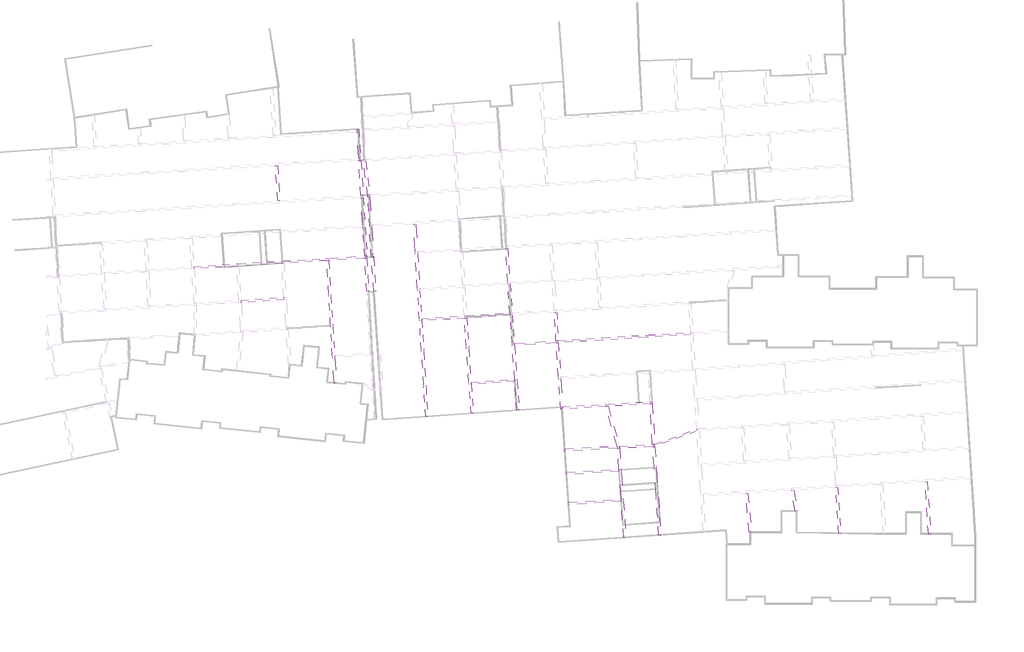
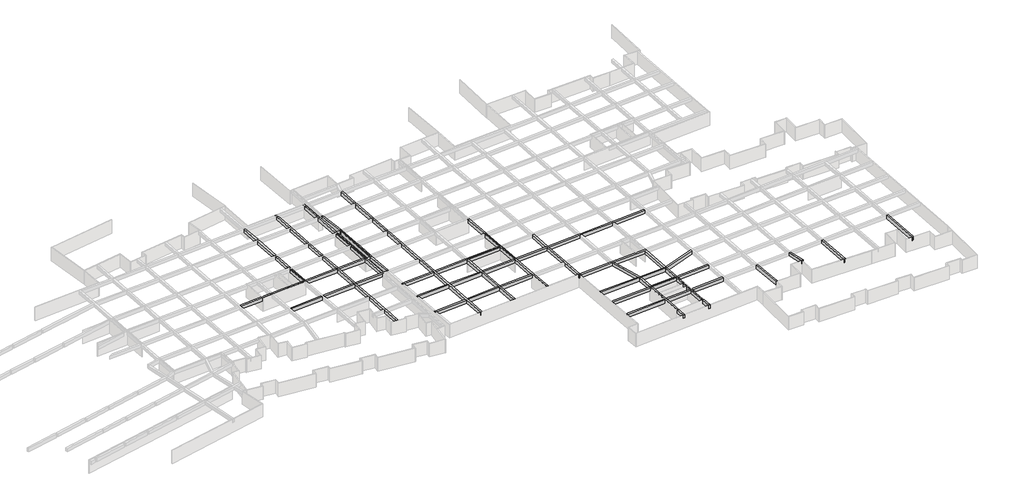
# One storey, part 12 of 14: 33 beams.
"""IFC4 building model written with IfcOpenShell, lengths in millimetres."""

from ifc_helpers import new_model, si_unit, frame, origin, place, context, project, spatial, polyline, outline, extrude, faceted_brep, element, save

model = new_model("IFC4")

# Units and contexts
model_context = context("Model", 3, world=origin())
ifc_project = project(units=[si_unit("LENGTHUNIT", "METRE", prefix="MILLI")], contexts=[model_context])

# Site, building, storey
site = spatial("IfcSite", under=ifc_project)
building = spatial("IfcBuilding", under=site)
storey = spatial("IfcBuildingStorey", under=building, Name="户型图", Elevation=0.0)

# Beams
placement = place(None, origin())
element("IfcBeam", 1, ObjectType="混凝土 - 矩形梁 : KL_beam", at=placement, inside=storey, context=model_context, shape_type="Brep", body=[
    faceted_brep([(-168844.3273357, -151421.9591856, 3300.0), (-168818.123542, -151821.1019553, 3300.0), (-161243.2908554, -151347.7846852, 3300.0), (-160844.0689153, -151322.8390994, 3300.0), (-153230.0656261, -150847.0742344, 3300.0), (-152830.8332777, -150822.1279982, 3300.0), (-145215.8086802, -150346.2993162, 3300.0), (-144816.5872887, -150321.3537646, 3300.0), (-138446.7291671, -149923.3299427, 3300.0), (-138047.4968186, -149898.3837065, 3300.0), (-138061.4513517, -149698.8245855, 3300.0), (-138075.4001739, -149499.3471348, 3300.0), (-138410.3239769, -149520.2750189, 3300.0), (-144841.5328402, -149922.1323731, 3300.0), (-145240.7542318, -149947.0779246, 3300.0), (-152857.2632096, -150422.9993589, 3300.0), (-153256.4846011, -150447.9449104, 3300.0), (-160869.6763174, -150923.659064, 3300.0), (-161268.8982576, -150948.6046498, 3300.0), (-138047.4968186, -149898.3837065, 2500.0), (-168818.123542, -151821.1019553, 2500.0), (-161243.2908554, -151347.7846852, 2500.0), (-160844.0689153, -151322.8390994, 2500.0), (-153230.0656261, -150847.0742344, 2500.0), (-152830.8332777, -150822.1279982, 2500.0), (-145215.8086802, -150346.2993162, 2500.0), (-144816.5872887, -150321.3537646, 2500.0), (-138446.7291671, -149923.3299427, 2500.0), (-168844.3273357, -151421.9591856, 2500.0), (-161268.8982576, -150948.6046498, 2500.0), (-160869.6763174, -150923.659064, 2500.0), (-153256.4846011, -150447.9449104, 2500.0), (-152857.2632096, -150422.9993589, 2500.0), (-145240.7542318, -149947.0779246, 2500.0), (-144841.5328402, -149922.1323731, 2500.0), (-138410.3239769, -149520.2750189, 2500.0), (-138075.4001739, -149499.3471348, 2500.0), (-138061.4513517, -149698.8245855, 2500.0)], [[[0, 1, 2, 3, 4, 5, 6, 7, 8, 9, 10, 11, 12, 13, 14, 15, 16, 17, 18]], [[19, 9, 8, 7, 6, 5, 4, 3, 2, 1, 20, 21, 22, 23, 24, 25, 26, 27]], [[20, 28, 29, 30, 31, 32, 33, 34, 35, 36, 37, 19, 27, 26, 25, 24, 23, 22, 21]], [[28, 0, 18, 17, 16, 15, 14, 13, 12, 11, 36, 35, 34, 33, 32, 31, 30, 29]], [[0, 28, 20, 1]], [[11, 10, 9, 19, 37, 36]]]),
])
element("IfcBeam", 2, ObjectType="混凝土 - 矩形梁 : KL_beam", at=placement, inside=storey, context=model_context, shape_type="SweptSolid", body=[
    extrude(outline(polyline([(-152857.2632096, -150422.9993589), (-153256.4846011, -150447.9449104), (-153570.081579, -145429.2295811), (-153170.8601875, -145404.2840296), (-152857.2632096, -150422.9993589)])), frame((0.0, 0.0, 2500.0), z_axis=(0.0, 0.0, 1.0), x_axis=(1.0, 0.0, 0.0)), (0.0, 0.0, 1.0), 800.0),
    extrude(outline(polyline([(-154632.6280549, -128424.5431139), (-154233.4066634, -128399.5975624), (-153944.0174942, -133030.8981222), (-154343.2012363, -133056.4462052), (-154632.6280549, -128424.5431139)])), frame((0.0, 0.0, 2500.0), z_axis=(0.0, 0.0, 1.0), x_axis=(1.0, 0.0, 0.0)), (0.0, 0.0, 1.0), 800.0),
    extrude(outline(polyline([(-153902.4547638, -140110.0252686), (-153503.2333722, -140085.079717), (-153195.805739, -145005.062638), (-153595.0271306, -145030.0081896), (-153902.4547638, -140110.0252686)])), frame((0.0, 0.0, 2500.0), z_axis=(0.0, 0.0, 1.0), x_axis=(1.0, 0.0, 0.0)), (0.0, 0.0, 1.0), 800.0),
    extrude(outline(polyline([(-153528.1789238, -139685.8583255), (-153927.4003153, -139710.803877), (-154318.2556563, -133455.6680514), (-153919.0719143, -133430.1199684), (-153528.1789238, -139685.8583255)])), frame((0.0, 0.0, 2500.0), z_axis=(0.0, 0.0, 1.0), x_axis=(1.0, 0.0, 0.0)), (0.0, 0.0, 1.0), 800.0),
])
element("IfcBeam", 3, ObjectType="混凝土 - 矩形梁 : KL_beam", at=placement, inside=storey, context=model_context, shape_type="Brep", body=[
    faceted_brep([(-143451.1806272, -172172.9270426, 3300.0), (-143850.4020187, -172197.8725942, 3300.0), (-143850.4020187, -172197.8725942, 2500.0), (-143451.1806272, -172172.9270426, 2500.0), (-143732.1819625, -167675.8629499, 3300.0), (-143757.1298345, -167276.6044225, 3300.0), (-144078.3820209, -162135.3773504, 3300.0), (-144103.3276067, -161736.1554102, 3300.0), (-144417.0732982, -156715.0601116, 3300.0), (-144442.0195344, -156315.8277631, 3300.0), (-144816.5872887, -150321.3537646, 3300.0), (-145215.8086802, -150346.2993162, 3300.0), (-144841.0561061, -156343.7311184, 3300.0), (-144816.1098699, -156742.9634669, 3300.0), (-144502.5076422, -161761.7628124, 3300.0), (-144477.5620564, -162160.9847526, 3300.0), (-144156.0109682, -167306.995361, 3300.0), (-144131.0630962, -167706.2538884, 3300.0), (-145215.8086802, -150346.2993162, 2500.0), (-144841.0561061, -156343.7311184, 2500.0), (-144816.1098699, -156742.9634669, 2500.0), (-144502.5076422, -161761.7628124, 2500.0), (-144477.5620564, -162160.9847526, 2500.0), (-144156.0109682, -167306.995361, 2500.0), (-144131.0630962, -167706.2538884, 2500.0), (-144816.5872887, -150321.3537646, 2500.0), (-144442.0195344, -156315.8277631, 2500.0), (-144417.0732982, -156715.0601116, 2500.0), (-144103.3276067, -161736.1554102, 2500.0), (-144078.3820209, -162135.3773504, 2500.0), (-143757.1298345, -167276.6044225, 2500.0), (-143732.1819625, -167675.8629499, 2500.0)], [[[0, 1, 2, 3]], [[1, 0, 4, 5, 6, 7, 8, 9, 10, 11, 12, 13, 14, 15, 16, 17]], [[2, 1, 17, 16, 15, 14, 13, 12, 11, 18, 19, 20, 21, 22, 23, 24]], [[3, 2, 24, 23, 22, 21, 20, 19, 18, 25, 26, 27, 28, 29, 30, 31]], [[0, 3, 31, 30, 29, 28, 27, 26, 25, 10, 9, 8, 7, 6, 5, 4]], [[11, 10, 25, 18]]]),
    faceted_brep([(-146252.6907928, -127338.3686664, 3300.0), (-146252.6907928, -127338.3686664, 2500.0), (-146651.9121843, -127363.3142179, 2500.0), (-146651.9121843, -127363.3142179, 3300.0), (-146242.6218456, -127499.509185, 3300.0), (-146641.8432371, -127524.4547366, 3300.0), (-146641.8432371, -127524.4547366, 2500.0), (-146242.6218456, -127499.509185, 2500.0)], [[[0, 1, 2, 3]], [[4, 5, 6, 7]], [[0, 3, 5, 4]], [[3, 2, 6, 5]], [[2, 1, 7, 6]], [[1, 0, 4, 7]]]),
    faceted_brep([(-144841.5328402, -149922.1323731, 3300.0), (-145240.7542318, -149947.0779246, 3300.0), (-145240.7542318, -149947.0779246, 2500.0), (-144841.5328402, -149922.1323731, 2500.0), (-145155.1298182, -144903.4170437, 3300.0), (-145554.3512097, -144928.3625953, 3300.0), (-145554.3512097, -144928.3625953, 2500.0), (-145155.1298182, -144903.4170437, 2500.0)], [[[0, 1, 2, 3]], [[1, 0, 4, 5]], [[2, 1, 5, 6]], [[3, 2, 6, 7]], [[0, 3, 7, 4]], [[5, 4, 7, 6]]]),
    faceted_brep([(-145886.7243944, -139609.1582827, 3300.0), (-145487.5030029, -139584.2127312, 3300.0), (-145487.5030029, -139584.2127312, 2500.0), (-145886.7243944, -139609.1582827, 2500.0), (-145180.0753697, -144504.1956522, 3300.0), (-145579.2967612, -144529.1412037, 3300.0), (-145579.2967612, -144529.1412037, 2500.0), (-145180.0753697, -144504.1956522, 2500.0)], [[[0, 1, 2, 3]], [[4, 5, 6, 7]], [[1, 0, 5, 4]], [[0, 3, 6, 5]], [[3, 2, 7, 6]], [[2, 1, 4, 7]]]),
    faceted_brep([(-145512.4485544, -139184.9913397, 3300.0), (-145911.669946, -139209.9368912, 3300.0), (-145911.669946, -139209.9368912, 2500.0), (-145512.4485544, -139184.9913397, 2500.0), (-145904.0974866, -132917.15511, 3300.0), (-146303.2812287, -132942.703193, 3300.0), (-146303.2812287, -132942.703193, 2500.0), (-145904.0974866, -132917.15511, 2500.0)], [[[0, 1, 2, 3]], [[1, 0, 4, 5]], [[2, 1, 5, 6]], [[3, 2, 6, 7]], [[0, 3, 7, 4]], [[5, 4, 7, 6]]]),
    faceted_brep([(-145929.0430666, -132517.9332638, 3300.0), (-146328.2268086, -132543.4813468, 3300.0), (-146328.2268086, -132543.4813468, 2500.0), (-145929.0430666, -132517.9332638, 2500.0), (-146217.676294, -127898.7305766, 3300.0), (-146616.8976856, -127923.6761281, 3300.0), (-146616.8976856, -127923.6761281, 2500.0), (-146217.676294, -127898.7305766, 2500.0)], [[[0, 1, 2, 3]], [[1, 0, 4, 5]], [[2, 1, 5, 6]], [[3, 2, 6, 7]], [[0, 3, 7, 4]], [[5, 4, 7, 6]]]),
])
element("IfcBeam", 4, ObjectType="混凝土 - 矩形梁 : KL_beam", at=placement, inside=storey, context=model_context, shape_type="Brep", body=[
    faceted_brep([(-137604.1419621, -156238.6535432, 3300.0), (-137632.0445516, -155839.6279231, 3300.0), (-138031.0701717, -155867.5305126, 3300.0), (-144442.0195344, -156315.8277631, 3300.0), (-144417.0732982, -156715.0601116, 3300.0), (-138005.1737883, -156266.6964203, 3300.0), (-137606.1281956, -156238.7924342, 3300.0), (-137604.1419621, -156238.6535432, 2500.0), (-144417.0732982, -156715.0601116, 2500.0), (-138005.1737883, -156266.6964203, 2500.0), (-137606.1281956, -156238.7924342, 2500.0), (-137632.0445516, -155839.6279231, 2500.0), (-144442.0195344, -156315.8277631, 2500.0), (-138031.0701717, -155867.5305126, 2500.0)], [[[0, 1, 2, 3, 4, 5, 6]], [[7, 0, 6, 5, 4, 8, 9, 10]], [[11, 7, 10, 9, 8, 12, 13]], [[1, 11, 13, 12, 3, 2]], [[4, 3, 12, 8]], [[1, 0, 7, 11]]]),
    faceted_brep([(-160426.3434263, -157834.5373332, 3300.0), (-160451.9512168, -157435.3512451, 3300.0), (-160451.9512168, -157435.3512451, 2500.0), (-160426.3434263, -157834.5373332, 2500.0), (-152806.7516024, -156900.7468094, 3300.0), (-152778.8490129, -157299.7724295, 3300.0), (-152778.8490129, -157299.7724295, 2500.0), (-152806.7516024, -156900.7468094, 2500.0)], [[[0, 1, 2, 3]], [[4, 5, 6, 7]], [[1, 0, 5, 4]], [[0, 3, 6, 5]], [[3, 2, 7, 6]], [[2, 1, 4, 7]]]),
    faceted_brep([(-152379.8233928, -157271.86984, 3300.0), (-152407.7259823, -156872.8442199, 3300.0), (-152407.7259823, -156872.8442199, 2500.0), (-152379.8233928, -157271.86984, 2500.0), (-144841.0561061, -156343.7311184, 3300.0), (-144816.1098699, -156742.9634669, 3300.0), (-144816.1098699, -156742.9634669, 2500.0), (-144841.0561061, -156343.7311184, 2500.0)], [[[0, 1, 2, 3]], [[4, 5, 6, 7]], [[1, 0, 5, 4]], [[0, 3, 6, 5]], [[3, 2, 7, 6]], [[2, 1, 4, 7]]]),
])
element("IfcBeam", 5, ObjectType="混凝土 - 矩形梁 : KL_beam", at=placement, inside=storey, context=model_context, shape_type="SweptSolid", body=[
    extrude(outline(polyline([(-139472.272293, -132525.1613278), (-139073.0509015, -132500.2157763), (-138682.0182996, -138758.1884339), (-139081.2396911, -138783.1339854), (-139472.272293, -132525.1613278)])), frame((0.0, 0.0, 2500.0), z_axis=(0.0, 0.0, 1.0), x_axis=(1.0, 0.0, 0.0)), (0.0, 0.0, 1.0), 800.0),
])
element("IfcBeam", 6, ObjectType="混凝土 - 矩形梁 : KL_beam", at=placement, inside=storey, context=model_context, shape_type="Brep", body=[
    faceted_brep([(-138257.4280169, -132256.5266916, 3300.0), (-138654.6809564, -132303.3252176, 3300.0), (-137889.4671884, -138798.902005, 3300.0), (-137866.6756453, -138992.369798, 3300.0), (-137478.1152384, -138968.0904035, 3300.0), (-137466.852736, -138967.3866603, 3300.0), (-137513.7217746, -138569.535169, 3300.0), (-138210.5692457, -132654.2910271, 3300.0), (-138654.6809564, -132303.3252176, 2500.0), (-137889.4671884, -138798.902005, 2500.0), (-137866.6756453, -138992.369798, 2500.0), (-138257.4280169, -132256.5266916, 2500.0), (-138210.5692457, -132654.2910271, 2500.0), (-137513.7217746, -138569.535169, 2500.0), (-137466.852736, -138967.3866603, 2500.0), (-137478.1152384, -138968.0904035, 2500.0)], [[[0, 1, 2, 3, 4, 5, 6, 7]], [[1, 8, 9, 10, 3, 2]], [[8, 11, 12, 13, 14, 15, 10, 9]], [[11, 0, 7, 6, 5, 14, 13, 12]], [[0, 11, 8, 1]], [[5, 4, 3, 10, 15, 14]]]),
])
element("IfcBeam", 7, ObjectType="混凝土 - 矩形梁 : KL_beam", at=placement, inside=storey, context=model_context, shape_type="SweptSolid", body=[
    extrude(outline(polyline([(-138446.7291671, -149923.3299427), (-138047.4968186, -149898.3837065), (-137632.0445516, -155839.6279231), (-138031.0701717, -155867.5305126), (-138446.7291671, -149923.3299427)])), frame((0.0, 0.0, 2500.0), z_axis=(0.0, 0.0, 1.0), x_axis=(1.0, 0.0, 0.0)), (0.0, 0.0, 1.0), 800.0),
])
element("IfcBeam", 8, ObjectType="混凝土 - 矩形梁 : KL_beam", at=placement, inside=storey, context=model_context, shape_type="Brep", body=[
    faceted_brep([(-136817.1755094, -149686.5252144, 3300.0), (-136817.1755094, -149686.5252144, 2500.0), (-137207.4432782, -149713.8153953, 2500.0), (-137216.2011295, -149714.4278039, 2500.0), (-137216.2011295, -149714.4278039, 3300.0), (-137207.4432782, -149713.8153953, 3300.0), (-136785.0174146, -155880.6422056, 3300.0), (-136385.9917945, -155852.7396161, 3300.0), (-136805.9297538, -149847.3470126, 3300.0), (-136785.0174146, -155880.6422056, 2500.0), (-136805.9297538, -149847.3470126, 2500.0), (-136385.9917945, -155852.7396161, 2500.0)], [[[0, 1, 2, 3, 4, 5]], [[0, 5, 4, 6, 7, 8]], [[4, 3, 9, 6]], [[3, 2, 1, 10, 11, 9]], [[1, 0, 8, 7, 11, 10]], [[7, 6, 9, 11]]]),
])
element("IfcBeam", 9, ObjectType="混凝土 - 矩形梁 : KL_beam", at=placement, inside=storey, context=model_context, shape_type="Brep", body=[
    faceted_brep([(-127144.4656282, -178152.7898071, 3300.0), (-127543.6605386, -178178.155601, 3300.0), (-127543.6605386, -178178.155601, 2500.0), (-127144.4656282, -178152.7898071, 2500.0), (-127473.8886953, -172968.4848239, 3300.0), (-127499.2550016, -172569.2818496, 3300.0), (-127884.2133482, -166510.9888115, 3300.0), (-127909.5791591, -166111.7936338, 3300.0), (-128228.3755197, -161094.7267499, 3300.0), (-128253.7413145, -160695.5318257, 3300.0), (-128570.7105944, -155707.2186766, 3300.0), (-128596.0769007, -155308.0157023, 3300.0), (-128988.5195114, -149131.9388421, 3300.0), (-129013.8853194, -148732.7437105, 3300.0), (-129323.5706608, -143859.0617527, 3300.0), (-129722.7922736, -143884.007318, 3300.0), (-129413.1069321, -148757.6892758, 3300.0), (-129387.7411242, -149156.8844074, 3300.0), (-128995.1105813, -155335.9188554, 3300.0), (-128969.744275, -155735.1218297, 3300.0), (-128652.9428893, -160720.7927378, 3300.0), (-128627.5770946, -161119.9876619, 3300.0), (-128308.8034239, -166136.6974613, 3300.0), (-128283.437613, -166535.892639, 3300.0), (-127898.2886822, -172597.1850027, 3300.0), (-127872.9223759, -172996.387977, 3300.0), (-129722.7922736, -143884.007318, 2500.0), (-129413.1069321, -148757.6892758, 2500.0), (-129387.7411242, -149156.8844074, 2500.0), (-128995.1105813, -155335.9188554, 2500.0), (-128969.744275, -155735.1218297, 2500.0), (-128652.9428893, -160720.7927378, 2500.0), (-128627.5770946, -161119.9876619, 2500.0), (-128308.8034239, -166136.6974613, 2500.0), (-128283.437613, -166535.892639, 2500.0), (-127898.2886822, -172597.1850027, 2500.0), (-127872.9223759, -172996.387977, 2500.0), (-129323.5706608, -143859.0617527, 2500.0), (-129013.8853194, -148732.7437105, 2500.0), (-128988.5195114, -149131.9388421, 2500.0), (-128596.0769007, -155308.0157023, 2500.0), (-128570.7105944, -155707.2186766, 2500.0), (-128253.7413145, -160695.5318257, 2500.0), (-128228.3755197, -161094.7267499, 2500.0), (-127909.5791591, -166111.7936338, 2500.0), (-127884.2133482, -166510.9888115, 2500.0), (-127499.2550016, -172569.2818496, 2500.0), (-127473.8886953, -172968.4848239, 2500.0)], [[[0, 1, 2, 3]], [[1, 0, 4, 5, 6, 7, 8, 9, 10, 11, 12, 13, 14, 15, 16, 17, 18, 19, 20, 21, 22, 23, 24, 25]], [[2, 1, 25, 24, 23, 22, 21, 20, 19, 18, 17, 16, 15, 26, 27, 28, 29, 30, 31, 32, 33, 34, 35, 36]], [[3, 2, 36, 35, 34, 33, 32, 31, 30, 29, 28, 27, 26, 37, 38, 39, 40, 41, 42, 43, 44, 45, 46, 47]], [[0, 3, 47, 46, 45, 44, 43, 42, 41, 40, 39, 38, 37, 14, 13, 12, 11, 10, 9, 8, 7, 6, 5, 4]], [[15, 14, 37, 26]]]),
    faceted_brep([(-130469.1405666, -132138.3296148, 3300.0), (-130070.0241354, -132111.7287526, 3300.0), (-130070.0241354, -132111.7287526, 2500.0), (-130469.1405666, -132138.3296148, 2500.0), (-129690.7407312, -138080.7122228, 3300.0), (-130089.9623439, -138105.6577881, 3300.0), (-130089.9623439, -138105.6577881, 2500.0), (-129690.7407312, -138080.7122228, 2500.0)], [[[0, 1, 2, 3]], [[4, 5, 6, 7]], [[1, 0, 5, 4]], [[0, 3, 6, 5]], [[3, 2, 7, 6]], [[2, 1, 4, 7]]]),
    faceted_brep([(-130095.3900507, -131712.5319316, 3300.0), (-130494.5064819, -131739.1327938, 3300.0), (-130494.5064819, -131739.1327938, 2500.0), (-130095.3900507, -131712.5319316, 2500.0), (-130407.3922508, -126802.388344, 3300.0), (-130806.6290639, -126827.0946929, 3300.0), (-130806.6290639, -126827.0946929, 2500.0), (-130407.3922508, -126802.388344, 2500.0)], [[[0, 1, 2, 3]], [[1, 0, 4, 5]], [[2, 1, 5, 6]], [[3, 2, 6, 7]], [[0, 3, 7, 4]], [[4, 7, 6, 5]]]),
    faceted_brep([(-130064.5965359, -138504.8529197, 3300.0), (-129665.3749232, -138479.9073544, 3300.0), (-129665.3749232, -138479.9073544, 2500.0), (-130064.5965359, -138504.8529197, 2500.0), (-129348.9364688, -143459.8666211, 3300.0), (-129748.1580815, -143484.8121864, 3300.0), (-129748.1580815, -143484.8121864, 2500.0), (-129348.9364688, -143459.8666211, 2500.0)], [[[0, 1, 2, 3]], [[4, 5, 6, 7]], [[1, 0, 5, 4]], [[0, 3, 6, 5]], [[3, 2, 7, 6]], [[2, 1, 4, 7]]]),
])
element("IfcBeam", 10, ObjectType="混凝土 - 矩形梁 : KL_beam", at=placement, inside=storey, context=model_context, shape_type="Brep", body=[
    faceted_brep([(-119455.2835342, -177579.9537582, 3300.0), (-119455.2835342, -177579.9537582, 2500.0), (-119056.2579141, -177552.0511687, 2500.0), (-119056.2579141, -177552.0511687, 3300.0), (-119416.172387, -172405.0344109, 3300.0), (-119444.0749765, -172006.0087908, 3300.0), (-119863.3119601, -166010.6406062, 3300.0), (-119891.2153372, -165611.6037233, 3300.0), (-120242.4030334, -160589.3856854, 3300.0), (-120641.613339, -160614.6471499, 3300.0), (-120290.4506032, -165636.508237, 3300.0), (-120262.5472261, -166035.54512, 3300.0), (-119843.1005966, -172033.9113803, 3300.0), (-119815.1980071, -172432.9370004, 3300.0), (-119416.172387, -172405.0344109, 2500.0), (-119444.0749765, -172006.0087908, 2500.0), (-119863.3119601, -166010.6406062, 2500.0), (-119891.2153372, -165611.6037233, 2500.0), (-120242.4030334, -160589.3856854, 2500.0), (-119815.1980071, -172432.9370004, 2500.0), (-119843.1005966, -172033.9113803, 2500.0), (-120262.5472261, -166035.54512, 2500.0), (-120290.4506032, -165636.508237, 2500.0), (-120641.613339, -160614.6471499, 2500.0)], [[[0, 1, 2, 3]], [[0, 3, 4, 5, 6, 7, 8, 9, 10, 11, 12, 13]], [[3, 2, 14, 15, 16, 17, 18, 8, 7, 6, 5, 4]], [[2, 1, 19, 20, 21, 22, 23, 18, 17, 16, 15, 14]], [[1, 0, 13, 12, 11, 10, 9, 23, 22, 21, 20, 19]], [[9, 8, 18, 23]]]),
])
element("IfcBeam", 11, ObjectType="混凝土 - 矩形梁 : KL_beam", at=placement, inside=storey, context=model_context, shape_type="Brep", body=[
    faceted_brep([(-110903.777801, -176972.188286, 3300.0), (-111302.8034211, -177000.0908755, 3300.0), (-111302.8034211, -177000.0908755, 2500.0), (-110903.777801, -176972.188286, 2500.0), (-111255.912427, -171936.4285221, 3300.0), (-111283.8160955, -171537.3874725, 3300.0), (-111705.867251, -165501.7747541, 3300.0), (-111733.7706281, -165102.7378711, 3300.0), (-112085.4797378, -160073.0632732, 3300.0), (-112113.3827977, -159674.0309265, 3300.0), (-112469.50037, -154581.3123772, 3300.0), (-112497.4029595, -154182.2867571, 3300.0), (-112920.7643368, -148127.9369941, 3300.0), (-113319.9966852, -148152.8832303, 3300.0), (-112896.4285796, -154210.1893466, 3300.0), (-112868.5259901, -154609.2149667, 3300.0), (-112512.581839, -159699.4534771, 3300.0), (-112484.6786383, -160098.4878378, 3300.0), (-112133.0058941, -165127.6423849, 3300.0), (-112105.102517, -165526.6792678, 3300.0), (-111689.9395138, -171463.7868185, 3300.0), (-111662.0369243, -171862.8124386, 3300.0), (-113319.9966852, -148152.8832303, 2500.0), (-112896.4285796, -154210.1893466, 2500.0), (-112868.5259901, -154609.2149667, 2500.0), (-112512.581839, -159699.4534771, 2500.0), (-112484.6786383, -160098.4878378, 2500.0), (-112133.0058941, -165127.6423849, 2500.0), (-112105.102517, -165526.6792678, 2500.0), (-111689.9395138, -171463.7868185, 2500.0), (-111662.0369243, -171862.8124386, 2500.0), (-112920.7643368, -148127.9369941, 2500.0), (-112497.4029595, -154182.2867571, 2500.0), (-112469.50037, -154581.3123772, 2500.0), (-112113.3827977, -159674.0309265, 2500.0), (-112085.4797378, -160073.0632732, 2500.0), (-111733.7706281, -165102.7378711, 2500.0), (-111705.867251, -165501.7747541, 2500.0), (-111283.8160955, -171537.3874725, 2500.0), (-111255.912427, -171936.4285221, 2500.0)], [[[0, 1, 2, 3]], [[1, 0, 4, 5, 6, 7, 8, 9, 10, 11, 12, 13, 14, 15, 16, 17, 18, 19, 20, 21]], [[2, 1, 21, 20, 19, 18, 17, 16, 15, 14, 13, 22, 23, 24, 25, 26, 27, 28, 29, 30]], [[3, 2, 30, 29, 28, 27, 26, 25, 24, 23, 22, 31, 32, 33, 34, 35, 36, 37, 38, 39]], [[0, 3, 39, 38, 37, 36, 35, 34, 33, 32, 31, 12, 11, 10, 9, 8, 7, 6, 5, 4]], [[13, 12, 31, 22]]]),
])
element("IfcBeam", 12, ObjectType="混凝土 - 矩形梁 : KL_beam", at=placement, inside=storey, context=model_context, shape_type="Brep", body=[
    faceted_brep([(-103469.2836775, -176821.0100704, 3300.0), (-103069.9236342, -176797.8899549, 3300.0), (-103097.8282277, -176398.8356759, 3300.0), (-103443.2472635, -171459.1133269, 3300.0), (-103471.1509319, -171060.0722772, 3300.0), (-103893.9013208, -165014.4600566, 3300.0), (-104293.1365867, -165039.3645704, 3300.0), (-103870.4219326, -171084.4657603, 3300.0), (-103842.5182642, -171483.50681, 3300.0), (-103069.9236342, -176797.8899549, 2500.0), (-103097.8282277, -176398.8356759, 2500.0), (-103443.2472635, -171459.1133269, 2500.0), (-103471.1509319, -171060.0722772, 2500.0), (-103893.9013208, -165014.4600566, 2500.0), (-103469.2836775, -176821.0100704, 2500.0), (-103842.5182642, -171483.50681, 2500.0), (-103870.4219326, -171084.4657603, 2500.0), (-104293.1365867, -165039.3645704, 2500.0)], [[[0, 1, 2, 3, 4, 5, 6, 7, 8]], [[1, 9, 10, 11, 12, 13, 5, 4, 3, 2]], [[9, 14, 15, 16, 17, 13, 12, 11, 10]], [[14, 0, 8, 7, 6, 17, 16, 15]], [[6, 5, 13, 17]], [[1, 0, 14, 9]]]),
])
element("IfcBeam", 13, ObjectType="混凝土 - 矩形梁 : KL_beam", at=placement, inside=storey, context=model_context, shape_type="SweptSolid", body=[
    extrude(outline(polyline([(-104584.7031482, -159592.3062757), (-104185.4951653, -159566.719321), (-103920.9067437, -164615.3671588), (-104320.1504642, -164640.2721999), (-104584.7031482, -159592.3062757)])), frame((0.0, 0.0, 2500.0), z_axis=(0.0, 0.0, 1.0), x_axis=(1.0, 0.0, 0.0)), (0.0, 0.0, 1.0), 800.0),
])
element("IfcBeam", 14, ObjectType="混凝土 - 矩形梁 : KL_beam", at=placement, inside=storey, context=model_context, shape_type="Brep", body=[
    faceted_brep([(-136436.7031727, -161213.3380996, 3300.0), (-136436.7031727, -161213.3380996, 2500.0), (-136411.4422615, -161612.5396606, 2500.0), (-136411.4422615, -161612.5396606, 3300.0), (-128652.9428893, -160720.7927378, 3300.0), (-128627.5770946, -161119.9876619, 3300.0), (-128627.5770946, -161119.9876619, 2500.0), (-128652.9428893, -160720.7927378, 2500.0), (-136384.3240936, -161610.8236612, 3300.0), (-135985.113788, -161585.5621967, 3300.0), (-136013.0169887, -161186.527836, 3300.0), (-136412.2272943, -161211.7893005, 3300.0), (-136384.3240936, -161610.8236612, 2500.0), (-135985.113788, -161585.5621967, 2500.0), (-136412.2272943, -161211.7893005, 2500.0), (-136013.0169887, -161186.527836, 2500.0)], [[[0, 1, 2, 3]], [[4, 5, 6, 7]], [[0, 3, 8, 9, 5, 4, 10, 11]], [[3, 2, 12, 13, 6, 5, 9, 8]], [[2, 1, 14, 15, 7, 6, 13, 12]], [[1, 0, 11, 10, 4, 7, 15, 14]]]),
    faceted_brep([(-112484.6786383, -160098.4878378, 3300.0), (-112512.581839, -159699.4534771, 3300.0), (-120265.8728019, -160190.0707833, 3300.0), (-120665.0977944, -160215.3331772, 3300.0), (-128253.7413145, -160695.5318257, 3300.0), (-128228.3755197, -161094.7267499, 3300.0), (-120641.613339, -160614.6471499, 3300.0), (-120242.4030334, -160589.3856854, 3300.0), (-112484.6786383, -160098.4878378, 2500.0), (-128228.3755197, -161094.7267499, 2500.0), (-120641.613339, -160614.6471499, 2500.0), (-120242.4030334, -160589.3856854, 2500.0), (-112512.581839, -159699.4534771, 2500.0), (-128253.7413145, -160695.5318257, 2500.0), (-120665.0977944, -160215.3331772, 2500.0), (-120265.8728019, -160190.0707833, 2500.0)], [[[0, 1, 2, 3, 4, 5, 6, 7]], [[8, 0, 7, 6, 5, 9, 10, 11]], [[12, 8, 11, 10, 9, 13, 14, 15]], [[1, 12, 15, 14, 13, 4, 3, 2]], [[1, 0, 8, 12]], [[5, 4, 13, 9]]]),
])
element("IfcBeam", 15, ObjectType="混凝土 - 矩形梁 : KL_beam", at=placement, inside=storey, context=model_context, shape_type="Brep", body=[
    faceted_brep([(-136058.4492738, -166620.1245981, 3300.0), (-136058.4492738, -166620.1245981, 2500.0), (-136033.545463, -167019.3485957, 2500.0), (-136033.545463, -167019.3485957, 3300.0), (-128308.8034239, -166136.6974613, 3300.0), (-128283.437613, -166535.892639, 3300.0), (-128283.437613, -166535.892639, 2500.0), (-128308.8034239, -166136.6974613, 2500.0), (-136006.242286, -167017.6454086, 3300.0), (-135607.0070201, -166992.7408948, 3300.0), (-135634.9103971, -166593.7040119, 3300.0), (-136034.1456631, -166618.6085256, 3300.0), (-136006.242286, -167017.6454086, 2500.0), (-135607.0070201, -166992.7408948, 2500.0), (-136034.1456631, -166618.6085256, 2500.0), (-135634.9103971, -166593.7040119, 2500.0)], [[[0, 1, 2, 3]], [[4, 5, 6, 7]], [[0, 3, 8, 9, 5, 4, 10, 11]], [[3, 2, 12, 13, 6, 5, 9, 8]], [[2, 1, 14, 15, 7, 6, 13, 12]], [[1, 0, 11, 10, 4, 7, 15, 14]]]),
    faceted_brep([(-111733.7706281, -165102.7378711, 3300.0), (-111705.867251, -165501.7747541, 3300.0), (-104293.1365867, -165039.3645704, 3300.0), (-103893.9013208, -165014.4600566, 3300.0), (-96247.3153136, -164537.461849, 3300.0), (-95848.0905559, -164512.5579908, 3300.0), (-88262.8201611, -164039.3846846, 3300.0), (-87863.5954035, -164014.4808264, 3300.0), (-80307.2636103, -163543.1127259, 3300.0), (-80332.7790985, -163143.9268851, 3300.0), (-87889.2782468, -163615.3054253, 3300.0), (-88288.5030044, -163640.2092835, 3300.0), (-95873.7733992, -164113.3825898, 3300.0), (-96272.9981569, -164138.286448, 3300.0), (-103920.9067437, -164615.3671588, 3300.0), (-104320.1504642, -164640.2721999, 3300.0), (-111705.867251, -165501.7747541, 2500.0), (-104293.1365867, -165039.3645704, 2500.0), (-103893.9013208, -165014.4600566, 2500.0), (-96247.3153136, -164537.461849, 2500.0), (-95848.0905559, -164512.5579908, 2500.0), (-88262.8201611, -164039.3846846, 2500.0), (-87863.5954035, -164014.4808264, 2500.0), (-80307.2636103, -163543.1127259, 2500.0), (-111733.7706281, -165102.7378711, 2500.0), (-104320.1504642, -164640.2721999, 2500.0), (-103920.9067437, -164615.3671588, 2500.0), (-96272.9981569, -164138.286448, 2500.0), (-95873.7733992, -164113.3825898, 2500.0), (-88288.5030044, -163640.2092835, 2500.0), (-87889.2782468, -163615.3054253, 2500.0), (-80332.7790985, -163143.9268851, 2500.0)], [[[0, 1, 2, 3, 4, 5, 6, 7, 8, 9, 10, 11, 12, 13, 14, 15]], [[1, 16, 17, 18, 19, 20, 21, 22, 23, 8, 7, 6, 5, 4, 3, 2]], [[16, 24, 25, 26, 27, 28, 29, 30, 31, 23, 22, 21, 20, 19, 18, 17]], [[24, 0, 15, 14, 13, 12, 11, 10, 9, 31, 30, 29, 28, 27, 26, 25]], [[1, 0, 24, 16]], [[9, 8, 23, 31]]]),
    faceted_brep([(-127884.2133482, -166510.9888115, 3300.0), (-127909.5791591, -166111.7936338, 3300.0), (-127909.5791591, -166111.7936338, 2500.0), (-127884.2133482, -166510.9888115, 2500.0), (-120290.4506032, -165636.508237, 3300.0), (-120262.5472261, -166035.54512, 3300.0), (-120262.5472261, -166035.54512, 2500.0), (-120290.4506032, -165636.508237, 2500.0)], [[[0, 1, 2, 3]], [[4, 5, 6, 7]], [[1, 0, 5, 4]], [[0, 3, 6, 5]], [[3, 2, 7, 6]], [[2, 1, 4, 7]]]),
    faceted_brep([(-119863.3119601, -166010.6406062, 3300.0), (-119891.2153372, -165611.6037233, 3300.0), (-119891.2153372, -165611.6037233, 2500.0), (-119863.3119601, -166010.6406062, 2500.0), (-112133.0058941, -165127.6423849, 3300.0), (-112105.102517, -165526.6792678, 3300.0), (-112105.102517, -165526.6792678, 2500.0), (-112133.0058941, -165127.6423849, 2500.0)], [[[0, 1, 2, 3]], [[4, 5, 6, 7]], [[1, 0, 5, 4]], [[0, 3, 6, 5]], [[3, 2, 7, 6]], [[2, 1, 4, 7]]]),
])
element("IfcBeam", 16, ObjectType="混凝土 - 矩形梁 : KL_beam", at=placement, inside=storey, context=model_context, shape_type="Brep", body=[
    faceted_brep([(-135604.5775407, -173136.0612145, 3300.0), (-135604.5775407, -173136.0612145, 2500.0), (-135576.6749512, -173535.0868346, 2500.0), (-135576.6749512, -173535.0868346, 3300.0), (-127898.2886822, -172597.1850027, 3300.0), (-127872.9223759, -172996.387977, 3300.0), (-127872.9223759, -172996.387977, 2500.0), (-127898.2886822, -172597.1850027, 2500.0), (-135550.6257594, -173533.2652977, 3300.0), (-135151.6001393, -173505.3627082, 3300.0), (-135179.5027288, -173106.3370881, 3300.0), (-135578.5283489, -173134.2396776, 3300.0), (-135550.6257594, -173533.2652977, 2500.0), (-135151.6001393, -173505.3627082, 2500.0), (-135578.5283489, -173134.2396776, 2500.0), (-135179.5027288, -173106.3370881, 2500.0)], [[[0, 1, 2, 3]], [[4, 5, 6, 7]], [[0, 3, 8, 9, 5, 4, 10, 11]], [[3, 2, 12, 13, 6, 5, 9, 8]], [[2, 1, 14, 15, 7, 6, 13, 12]], [[1, 0, 11, 10, 4, 7, 15, 14]]]),
    faceted_brep([(-127499.2550016, -172569.2818496, 3300.0), (-127473.8886953, -172968.4848239, 3300.0), (-119815.1980071, -172432.9370004, 3300.0), (-119843.1005966, -172033.9113803, 3300.0), (-127473.8886953, -172968.4848239, 2500.0), (-119815.1980071, -172432.9370004, 2500.0), (-127499.2550016, -172569.2818496, 2500.0), (-119843.1005966, -172033.9113803, 2500.0)], [[[0, 1, 2, 3]], [[1, 4, 5, 2]], [[4, 6, 7, 5]], [[6, 0, 3, 7]], [[1, 0, 6, 4]], [[3, 2, 5, 7]]]),
    faceted_brep([(-111689.9395138, -171463.7868185, 3300.0), (-111662.0369243, -171862.8124386, 3300.0), (-111662.0369243, -171862.8124386, 2500.0), (-111689.9395138, -171463.7868185, 2500.0), (-119416.172387, -172405.0344109, 3300.0), (-119444.0749765, -172006.0087908, 3300.0), (-119444.0749765, -172006.0087908, 2500.0), (-119416.172387, -172405.0344109, 2500.0)], [[[0, 1, 2, 3]], [[4, 5, 6, 7]], [[1, 0, 5, 4]], [[2, 1, 4, 7]], [[3, 2, 7, 6]], [[0, 3, 6, 5]]]),
])
element("IfcBeam", 17, ObjectType="混凝土 - 矩形梁 : KL_beam", at=placement, inside=storey, context=model_context, shape_type="Brep", body=[
    faceted_brep([(-87136.5215317, -175875.4589234, 3300.0), (-87136.6712903, -175872.8721019, 3300.0), (-87159.6399867, -175476.127561, 3300.0), (-87558.9713492, -175499.2460161, 3300.0), (-95113.0722271, -175936.5749066, 3300.0), (-95512.4118264, -175959.6938385, 3300.0), (-103097.8282277, -176398.8356759, 3300.0), (-103069.9236342, -176797.8899549, 3300.0), (-95448.0556935, -176356.6378318, 3300.0), (-95038.7309253, -176332.9408294, 3300.0), (-87535.8528941, -175898.5773785, 3300.0), (-87136.5215317, -175875.4589234, 2500.0), (-103069.9236342, -176797.8899549, 2500.0), (-95448.0556935, -176356.6378318, 2500.0), (-95038.7309253, -176332.9408294, 2500.0), (-87535.8528941, -175898.5773785, 2500.0), (-87159.6399867, -175476.127561, 2500.0), (-87136.6712903, -175872.8721019, 2500.0), (-103097.8282277, -176398.8356759, 2500.0), (-95512.4118264, -175959.6938385, 2500.0), (-95113.0722271, -175936.5749066, 2500.0), (-87558.9713492, -175499.2460161, 2500.0)], [[[0, 1, 2, 3, 4, 5, 6, 7, 8, 9, 10]], [[11, 0, 10, 9, 8, 7, 12, 13, 14, 15]], [[16, 17, 11, 15, 14, 13, 12, 18, 19, 20, 21]], [[2, 16, 21, 20, 19, 18, 6, 5, 4, 3]], [[7, 6, 18, 12]], [[2, 1, 0, 11, 17, 16]]]),
])
element("IfcBeam", 18, ObjectType="混凝土 - 矩形梁 : KL_beam", at=placement, inside=storey, context=model_context, shape_type="Brep", body=[
    faceted_brep([(-93298.3309579, -183853.6189251, 3300.0), (-92946.2984043, -183835.1696807, 3300.0), (-92888.3719204, -183832.1338823, 3300.0), (-93001.5270207, -183437.5151514, 3300.0), (-95038.7309253, -176332.9408294, 3300.0), (-95448.0556935, -176356.6378318, 3300.0), (-93424.864736, -183412.3431998, 3300.0), (-93311.7096358, -183806.9619306, 3300.0), (-93298.3309579, -183853.6189251, 2500.0), (-95448.0556935, -176356.6378318, 2500.0), (-93424.864736, -183412.3431998, 2500.0), (-93311.7096358, -183806.9619306, 2500.0), (-92888.3719204, -183832.1338823, 2500.0), (-92946.2984043, -183835.1696807, 2500.0), (-95038.7309253, -176332.9408294, 2500.0), (-93001.5270207, -183437.5151514, 2500.0)], [[[0, 1, 2, 3, 4, 5, 6, 7]], [[8, 0, 7, 6, 5, 9, 10, 11]], [[12, 13, 8, 11, 10, 9, 14, 15]], [[2, 12, 15, 14, 4, 3]], [[5, 4, 14, 9]], [[2, 1, 0, 8, 13, 12]]]),
])
element("IfcBeam", 19, ObjectType="混凝土 - 矩形梁 : KL_beam", at=placement, inside=storey, context=model_context, shape_type="Brep", body=[
    faceted_brep([(-86718.3835388, -183508.778493, 3300.0), (-86799.0163949, -183112.4553436, 3300.0), (-87117.2549502, -183129.1335195, 3300.0), (-93001.5270207, -183437.5151514, 3300.0), (-92888.3719204, -183832.1338823, 3300.0), (-87091.7695674, -183528.3468256, 3300.0), (-86718.3835388, -183508.778493, 2500.0), (-92888.3719205, -183832.1338823, 2500.0), (-87091.7695674, -183528.3468256, 2500.0), (-86799.0163949, -183112.4553436, 2500.0), (-93001.5270207, -183437.5151514, 2500.0), (-87117.2549502, -183129.1335195, 2500.0)], [[[0, 1, 2, 3, 4, 5]], [[6, 0, 5, 4, 7, 8]], [[9, 6, 8, 7, 10, 11]], [[1, 9, 11, 10, 3, 2]], [[4, 3, 10, 7]], [[1, 0, 6, 9]]]),
])
element("IfcBeam", 20, ObjectType="混凝土 - 矩形梁 : KL_beam", at=placement, inside=storey, context=model_context, shape_type="Brep", body=[
    faceted_brep([(-86799.0163949, -183112.4553436, 3300.0), (-86718.3835388, -183508.778493, 3300.0), (-86692.811988, -183499.4712097, 3300.0), (-79205.8573257, -180774.4425673, 3300.0), (-79232.4471215, -180358.4493525, 3300.0), (-86719.2319039, -183083.4161637, 3300.0), (-86718.3835388, -183508.778493, 2500.0), (-86692.811988, -183499.4712097, 2500.0), (-79205.8573257, -180774.4425673, 2500.0), (-86799.0163949, -183112.4553436, 2500.0), (-86719.2319039, -183083.4161637, 2500.0), (-79232.4471215, -180358.4493525, 2500.0)], [[[0, 1, 2, 3, 4, 5]], [[1, 6, 7, 8, 3, 2]], [[6, 9, 10, 11, 8, 7]], [[9, 0, 5, 4, 11, 10]], [[0, 9, 6, 1]], [[4, 3, 8, 11]]]),
])
element("IfcBeam", 21, ObjectType="混凝土 - 矩形梁 : KL_beam", at=placement, inside=storey, context=model_context, shape_type="SweptSolid", body=[
    extrude(outline(polyline([(-87535.8528941, -175898.5773785), (-87136.5215317, -175875.4589234), (-86719.2319039, -183083.4161637), (-86799.0163949, -183112.4553436), (-87117.2549502, -183129.1335195), (-87535.8528941, -175898.5773785)])), frame((0.0, 0.0, 2500.0), z_axis=(0.0, 0.0, 1.0), x_axis=(1.0, 0.0, 0.0)), (0.0, 0.0, 1.0), 800.0),
])
element("IfcBeam", 22, ObjectType="混凝土 - 矩形梁 : KL_beam", at=placement, inside=storey, context=model_context, shape_type="Brep", body=[
    faceted_brep([(-102769.8718668, -183902.0942709, 3300.0), (-102769.8718668, -183902.0942709, 2500.0), (-102748.9374843, -184301.5460848, 2500.0), (-102748.9374843, -184301.5460848, 3300.0), (-93349.110578, -183808.922031, 3300.0), (-93311.7096358, -183806.9619306, 3300.0), (-93411.4860581, -183459.0001942, 3300.0), (-93424.864736, -183412.3431998, 3300.0), (-93349.110578, -183808.922031, 2500.0), (-93311.7096358, -183806.9619306, 2500.0), (-93424.864736, -183412.3431998, 2500.0), (-93411.4860581, -183459.0001942, 2500.0)], [[[0, 1, 2, 3]], [[0, 3, 4, 5, 6, 7]], [[3, 2, 8, 9, 5, 4]], [[2, 1, 10, 11, 9, 8]], [[1, 0, 7, 10]], [[5, 9, 11, 10, 7, 6]]]),
])
element("IfcBeam", 23, ObjectType="混凝土 - 矩形梁 : KL_beam", at=placement, inside=storey, context=model_context, shape_type="Brep", body=[
    faceted_brep([(-91834.2142361, -199738.7142198, 3300.0), (-92233.2398562, -199766.6168093, 3300.0), (-92233.2398562, -199766.6168093, 2500.0), (-91834.2142361, -199738.7142198, 2500.0), (-92289.1828809, -193232.3594737, 3300.0), (-92317.0859695, -192833.326716, 3300.0), (-92663.0775802, -187885.4161643, 3300.0), (-92690.9806688, -187486.3834066, 3300.0), (-92946.2984043, -183835.1696807, 3300.0), (-93298.3309579, -183853.6189251, 3300.0), (-93311.7096358, -183806.9619306, 3300.0), (-93349.110578, -183808.922031, 3300.0), (-93090.1731814, -187511.8993213, 3300.0), (-93062.2700928, -187910.932079, 3300.0), (-92716.2784822, -192858.8426307, 3300.0), (-92688.3753936, -193257.8753884, 3300.0), (-93349.110578, -183808.922031, 2500.0), (-93090.1731814, -187511.8993213, 2500.0), (-93062.2700928, -187910.932079, 2500.0), (-92716.2784822, -192858.8426307, 2500.0), (-92688.3753936, -193257.8753884, 2500.0), (-93311.7096358, -183806.9619306, 2500.0), (-93298.3309579, -183853.6189251, 2500.0), (-92946.2984043, -183835.1696807, 2500.0), (-92690.9806688, -187486.3834066, 2500.0), (-92663.0775802, -187885.4161643, 2500.0), (-92317.0859695, -192833.326716, 2500.0), (-92289.1828809, -193232.3594737, 2500.0)], [[[0, 1, 2, 3]], [[1, 0, 4, 5, 6, 7, 8, 9, 10, 11, 12, 13, 14, 15]], [[2, 1, 15, 14, 13, 12, 11, 16, 17, 18, 19, 20]], [[3, 2, 20, 19, 18, 17, 16, 21, 22, 23, 24, 25, 26, 27]], [[0, 3, 27, 26, 25, 24, 23, 8, 7, 6, 5, 4]], [[16, 11, 10, 21]], [[9, 22, 21, 10]], [[22, 9, 8, 23]]]),
])
element("IfcBeam", 24, ObjectType="混凝土 - 矩形梁 : KL_beam", at=placement, inside=storey, context=model_context, shape_type="Brep", body=[
    faceted_brep([(-85585.375515, -199336.5506095, 3300.0), (-85984.4011351, -199364.453199, 3300.0), (-85984.4011351, -199364.453199, 2500.0), (-85585.375515, -199336.5506095, 2500.0), (-86040.1530504, -192832.9288557, 3300.0), (-86068.056139, -192433.896098, 3300.0), (-86414.0477496, -187485.9855463, 3300.0), (-86441.9508382, -187086.9527886, 3300.0), (-86692.811988, -183499.4712097, 3300.0), (-86695.0971155, -183500.3029281, 3300.0), (-86718.3835388, -183508.778493, 3300.0), (-87091.7695674, -183528.3468256, 3300.0), (-86841.1433509, -187112.4687033, 3300.0), (-86813.2402623, -187511.501461, 3300.0), (-86467.2486516, -192459.4120127, 3300.0), (-86439.345563, -192858.4447704, 3300.0), (-87091.7695674, -183528.3468256, 2500.0), (-86841.1433509, -187112.4687033, 2500.0), (-86813.2402623, -187511.501461, 2500.0), (-86467.2486516, -192459.4120127, 2500.0), (-86439.345563, -192858.4447704, 2500.0), (-86718.3835388, -183508.778493, 2500.0), (-86695.0971155, -183500.3029281, 2500.0), (-86692.811988, -183499.4712097, 2500.0), (-86441.9508382, -187086.9527886, 2500.0), (-86414.0477496, -187485.9855463, 2500.0), (-86068.056139, -192433.896098, 2500.0), (-86040.1530504, -192832.9288557, 2500.0)], [[[0, 1, 2, 3]], [[1, 0, 4, 5, 6, 7, 8, 9, 10, 11, 12, 13, 14, 15]], [[2, 1, 15, 14, 13, 12, 11, 16, 17, 18, 19, 20]], [[3, 2, 20, 19, 18, 17, 16, 21, 22, 23, 24, 25, 26, 27]], [[0, 3, 27, 26, 25, 24, 23, 8, 7, 6, 5, 4]], [[11, 10, 21, 16]], [[8, 23, 22, 21, 10, 9]]]),
])
element("IfcBeam", 25, ObjectType="混凝土 - 矩形梁 : KL_beam", at=placement, inside=storey, context=model_context, shape_type="SweptSolid", body=[
    extrude(outline(polyline([(-102452.1145409, -188511.1198638), (-102477.6299992, -188111.9344916), (-93090.1731814, -187511.8993213), (-93062.2700928, -187910.932079), (-102452.1145409, -188511.1198638)])), frame((0.0, 0.0, 2500.0), z_axis=(0.0, 0.0, 1.0), x_axis=(1.0, 0.0, 0.0)), (0.0, 0.0, 1.0), 800.0),
    extrude(outline(polyline([(-92663.0775802, -187885.4161643), (-92690.9806688, -187486.3834066), (-86841.1433509, -187112.4687033), (-86813.2402623, -187511.501461), (-92663.0775802, -187885.4161643)])), frame((0.0, 0.0, 2500.0), z_axis=(0.0, 0.0, 1.0), x_axis=(1.0, 0.0, 0.0)), (0.0, 0.0, 1.0), 800.0),
    extrude(outline(polyline([(-78833.4545077, -186600.626675), (-78807.9390495, -186999.8120473), (-86414.0477496, -187485.9855463), (-86441.9508382, -187086.9527886), (-78833.4545077, -186600.626675)])), frame((0.0, 0.0, 2500.0), z_axis=(0.0, 0.0, 1.0), x_axis=(1.0, 0.0, 0.0)), (0.0, 0.0, 1.0), 800.0),
])
element("IfcBeam", 26, ObjectType="混凝土 - 矩形梁 : KL_beam", at=placement, inside=storey, context=model_context, shape_type="SweptSolid", body=[
    extrude(outline(polyline([(-102078.2492638, -193858.0650538), (-102103.7647221, -193458.8796816), (-92716.2784822, -192858.8426307), (-92688.3753936, -193257.8753884), (-102078.2492638, -193858.0650538)])), frame((0.0, 0.0, 2500.0), z_axis=(0.0, 0.0, 1.0), x_axis=(1.0, 0.0, 0.0)), (0.0, 0.0, 1.0), 800.0),
    extrude(outline(polyline([(-92289.1828809, -193232.3594737), (-92317.0859695, -192833.326716), (-86467.2486516, -192459.4120127), (-86439.345563, -192858.4447704), (-92289.1828809, -193232.3594737)])), frame((0.0, 0.0, 2500.0), z_axis=(0.0, 0.0, 1.0), x_axis=(1.0, 0.0, 0.0)), (0.0, 0.0, 1.0), 800.0),
    extrude(outline(polyline([(-78491.5534826, -191949.6149824), (-78466.0380243, -192348.8003546), (-86040.1530504, -192832.9288557), (-86068.056139, -192433.896098), (-78491.5534826, -191949.6149824)])), frame((0.0, 0.0, 2500.0), z_axis=(0.0, 0.0, 1.0), x_axis=(1.0, 0.0, 0.0)), (0.0, 0.0, 1.0), 800.0),
])
element("IfcBeam", 27, ObjectType="混凝土 - 矩形梁 : KL_beam", at=placement, inside=storey, context=model_context, shape_type="SweptSolid", body=[
    extrude(outline(polyline([(-69491.0878234, -198749.6229603), (-69889.5657027, -198784.4852574), (-70497.8882735, -191831.3264562), (-70098.6297483, -191805.3869831), (-69491.0878234, -198749.6229603)])), frame((0.0, 0.0, 2500.0), z_axis=(0.0, 0.0, 1.0), x_axis=(1.0, 0.0, 0.0)), (0.0, 0.0, 1.0), 800.0),
])
element("IfcBeam", 28, ObjectType="混凝土 - 矩形梁 : KL_beam", at=placement, inside=storey, context=model_context, shape_type="SweptSolid", body=[
    extrude(outline(polyline([(-61244.3150773, -194974.7527087), (-61636.6478024, -195052.6952056), (-62381.3788239, -191304.0040188), (-61978.7583486, -191277.8461227), (-61244.3150773, -194974.7527087)])), frame((0.0, 0.0, 2500.0), z_axis=(0.0, 0.0, 1.0), x_axis=(1.0, 0.0, 0.0)), (0.0, 0.0, 1.0), 800.0),
])
element("IfcBeam", 29, ObjectType="混凝土 - 矩形梁 : KL_beam", at=placement, inside=storey, context=model_context, shape_type="SweptSolid", body=[
    extrude(outline(polyline([(-53516.0609997, -199003.4775051), (-53915.2194657, -199029.4104774), (-54450.6079601, -190788.7488529), (-54051.4494941, -190762.8158805), (-53516.0609997, -199003.4775051)])), frame((0.0, 0.0, 2500.0), z_axis=(0.0, 0.0, 1.0), x_axis=(1.0, 0.0, 0.0)), (0.0, 0.0, 1.0), 800.0),
])
element("IfcBeam", 30, ObjectType="混凝土 - 矩形梁 : KL_beam", at=placement, inside=storey, context=model_context, shape_type="SweptSolid", body=[
    extrude(outline(polyline([(-37518.4612868, -199115.8810931), (-37917.6197528, -199141.8140654), (-38527.5221301, -189754.2400553), (-38128.3636641, -189728.3070829), (-37518.4612868, -199115.8810931)])), frame((0.0, 0.0, 2500.0), z_axis=(0.0, 0.0, 1.0), x_axis=(1.0, 0.0, 0.0)), (0.0, 0.0, 1.0), 800.0),
])
element("IfcBeam", 31, ObjectType="混凝土 - 矩形梁 : KL_beam", at=placement, inside=storey, context=model_context, shape_type="Brep", body=[
    faceted_brep([(-137998.6323624, -149694.899309, 2500.0), (-137998.6323624, -149694.899309, 3300.0), (-138061.4513517, -149698.8245855, 3300.0), (-138061.4513517, -149698.8245855, 2500.0), (-138657.072748, -139157.4098254, 3300.0), (-139056.2941396, -139182.355377, 3300.0), (-138748.8665064, -144102.338298, 3300.0), (-138723.9209548, -144501.5596895, 3300.0), (-138410.3239769, -149520.2750189, 3300.0), (-138075.4001739, -149499.3471348, 3300.0), (-139056.2941396, -139182.355377, 2500.0), (-138748.8665064, -144102.338298, 2500.0), (-138723.9209548, -144501.5596895, 2500.0), (-138410.3239769, -149520.2750189, 2500.0), (-138657.072748, -139157.4098254, 2500.0), (-138075.4001739, -149499.3471348, 2500.0)], [[[0, 1, 2, 3]], [[1, 4, 5, 6, 7, 8, 9, 2]], [[5, 10, 11, 12, 13, 8, 7, 6]], [[14, 0, 3, 15, 13, 12, 11, 10]], [[1, 0, 14, 4]], [[5, 4, 14, 10]], [[15, 9, 8, 13]], [[9, 15, 3, 2]]]),
])
element("IfcBeam", 32, ObjectType="混凝土 - 矩形梁 : KL_beam", at=placement, inside=storey, context=model_context, shape_type="Brep", body=[
    faceted_brep([(-136798.3489589, -149846.8733228, 2500.0), (-136798.3489589, -149846.8733228, 3300.0), (-136805.9297538, -149847.3470126, 3300.0), (-136805.9297538, -149847.3470126, 2500.0), (-137866.6756453, -138992.369798, 3300.0), (-137889.4671884, -138798.902005, 3300.0), (-137207.4432782, -149713.8153953, 3300.0), (-136817.1755094, -149686.5252144, 3300.0), (-136812.4738529, -149620.8226053, 3300.0), (-137020.4840836, -149633.8202303, 3300.0), (-137045.4296351, -149234.5988387, 3300.0), (-136837.4194044, -149221.6012138, 3300.0), (-137141.9739314, -144347.5986544, 3300.0), (-137166.9194829, -143948.3772629, 3300.0), (-137478.1152384, -138968.0904035, 3300.0), (-137889.4671884, -138798.902005, 2500.0), (-137207.4432782, -149713.8153953, 2500.0), (-137866.6756453, -138992.369798, 2500.0), (-137478.1152384, -138968.0904035, 2500.0), (-137166.9194829, -143948.3772629, 2500.0), (-137141.9739314, -144347.5986544, 2500.0), (-136837.4194044, -149221.6012138, 2500.0), (-137045.4296351, -149234.5988387, 2500.0), (-137020.4840836, -149633.8202303, 2500.0), (-136812.4738529, -149620.8226053, 2500.0), (-136817.1755094, -149686.5252144, 2500.0)], [[[0, 1, 2, 3]], [[4, 5, 6, 7, 2, 1, 8, 9, 10, 11, 12, 13, 14]], [[5, 15, 16, 6]], [[15, 17, 18, 19, 20, 21, 22, 23, 24, 0, 3, 25, 16]], [[1, 0, 24, 8]], [[4, 17, 15, 5]], [[17, 4, 14, 18]], [[25, 7, 6, 16]], [[7, 25, 3, 2]], [[22, 10, 9, 23]], [[23, 9, 8, 24]], [[10, 22, 21, 11]], [[18, 14, 13, 12, 11, 21, 20, 19]]]),
])
element("IfcBeam", 33, ObjectType="混凝土 - 矩形梁 : KL_beam", at=placement, inside=storey, context=model_context, shape_type="SweptSolid", body=[
    extrude(outline(polyline([(-139821.4700239, -126936.7018456), (-139422.2486323, -126911.7562941), (-139073.0509015, -132500.2157763), (-139472.272293, -132525.1613278), (-139473.4951331, -132505.5913482), (-139271.5629231, -132492.6675232), (-139297.110977, -132093.4842358), (-139498.4407131, -132106.369502), (-139786.4674307, -127496.8732223), (-139718.9450314, -127492.6540509), (-139743.8905829, -127093.4326594), (-139811.4129822, -127097.6518308), (-139821.4700239, -126936.7018456)])), frame((0.0, 0.0, 2500.0), z_axis=(0.0, 0.0, 1.0), x_axis=(1.0, 0.0, 0.0)), (0.0, 0.0, 1.0), 800.0),
])

save(model, "model.ifc")

# Revit data of these elements
# Type "混凝土 - 矩形梁 : KL_beam"
#   Length [instance default] = 1524 mm
#   b = 400 mm
#   h = 800 mm
#   Structural Material [instance default] = 混凝土 - 现场浇注混凝土
#   Assembly Code = ""
# Elements 1, 2, 3, 4, 5, 6, 7, 8, 9, 10, 11, 12, 13, 14, 15, 16, 17, 18, 19, 20, 21, 22, 23, 24, 25, 26, 27, 28, 29, 30, 31, 32, 33 (IfcBeam, "混凝土 - 矩形梁 : KL_beam")
#   Comments = ""
#   Structural Material = none
#   Phase Created = 新构造
# Materials
#   "混凝土 - 现场浇注混凝土": class "混凝土", colour RGB 192 192 192, transparency 0
